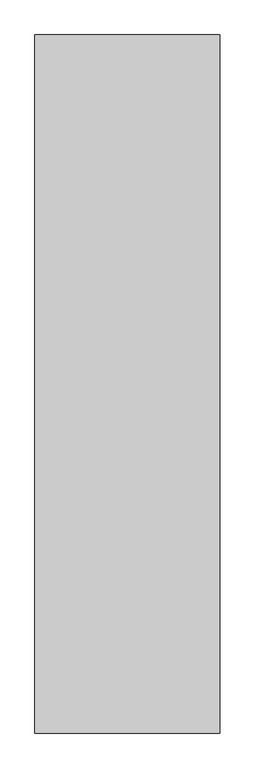
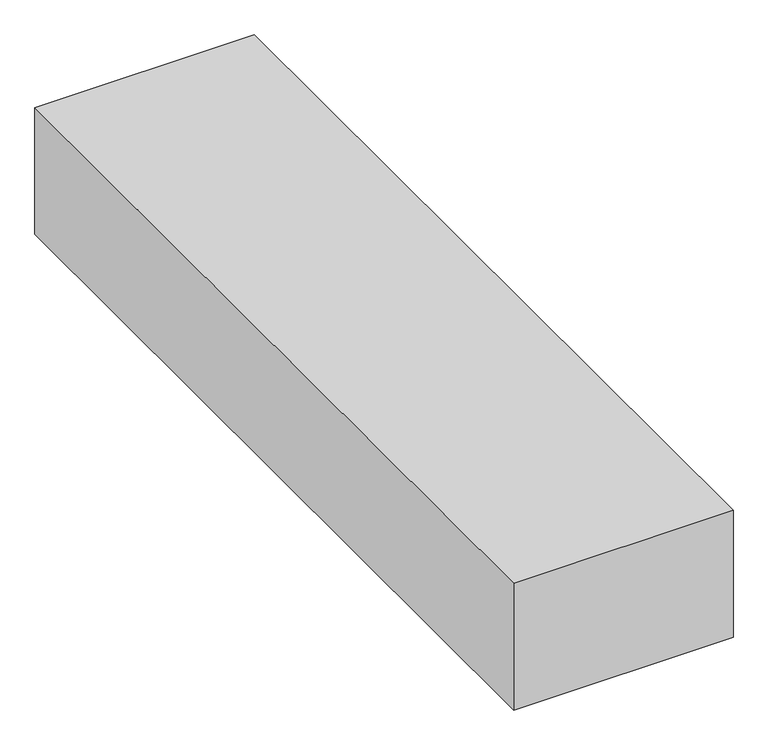
"""IFC4 building model written with IfcOpenShell, lengths in millimetres: proxy geometry, Space Planning Box_hec : Space Planning Box_hec."""

from ifc_helpers import new_model, si_unit, origin, origin_with_axes, place, context, project, spatial, polyline, outline, extrude, source, transform, mapped, element, save


def generic_models_8b5775ea(model_context):
    return source(origin(), model_context, "Body", "SweptSolid", [
        extrude(outline(polyline([(4500.0, 17000.0), (4500.0, -17000.0), (-4500.0, -17000.0), (-4500.0, 17000.0), (4500.0, 17000.0)])), origin_with_axes(), (0.0, 0.0, 1.0), 5500.0),
    ])


if __name__ == "__main__":
    model = new_model("IFC4")
    model_context = context("Model", 3, world=origin())
    ifc_project = project(units=[si_unit("LENGTHUNIT", "METRE", prefix="MILLI")], contexts=[model_context])
    site = spatial("IfcSite", under=ifc_project)
    building = spatial("IfcBuilding", under=site)
    placement = place(None, origin())
    generic_models_shape = generic_models_8b5775ea(model_context)
    element("IfcBuildingElementProxy", 1, Name="Space Planning Box_hec : Space Planning Box_hec", ObjectType="Space Planning Box_hec : Space Planning Box_hec", at=placement, inside=building, context=model_context, shape_type="MappedRepresentation", body=[
        mapped(generic_models_shape, transform((0.0, 0.0, 0.0), x_axis=(1.0, 0.0, 0.0), y_axis=(0.0, 1.0, 0.0), z_axis=(0.0, 0.0, 1.0))),
    ])
    save(model, "model.ifc")

# Revit data of these elements
# Type "Space Planning Box_hec : Space Planning Box_hec"
#   Type Comments = "..."
#   Room Name [instance default] = "?"
#   Interior Finish [instance default] = ""
#   Exterior Finish [instance default] = ""
#   Department [instance default] = ""
#   Assembly Code = "..."
#   ceiling height [instance default] = 0
#   Width [instance default] = 1524 mm
#   Program Area [instance default] = 0.00 m²
#   Length [instance default] = 1524 mm
#   Height [instance default] = 1524 mm
#   Area [instance default] = 2.32258 m²
#   Fill Color [instance default] = Cyan
#   Default Elevation = 0
# Element 1 (IfcBuildingElementProxy, "Space Planning Box_hec : Space Planning Box_hec")
#   Room Name = "Electrical Room-2"
#   Exterior Finish = "N/A..N/A,,EW1..EW2..N/A"
#   Department = "EL"
#   Width = 9000 mm
#   Program Area = 288.00 m²
#   Length = 34000 mm
#   Height = 5500 mm
#   Area = 306.00 m²
#   Fill Color = Orange
#   Materials on its faces: "Orange"
# Materials
#   "Cyan": class "Generic", colour RGB 0 255 255, transparency 0.2, Cost = 0
#   "Orange": class "Generic", colour RGB 255 165 0, transparency 0.2, Cost = 0
